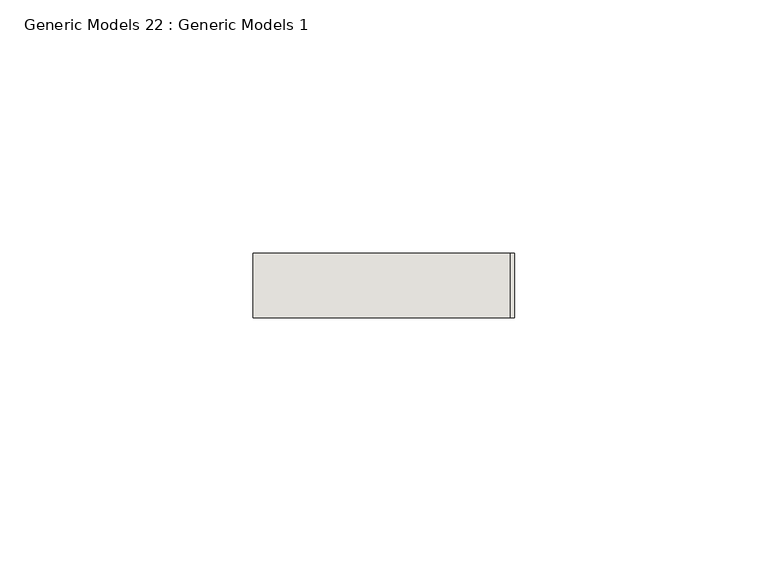
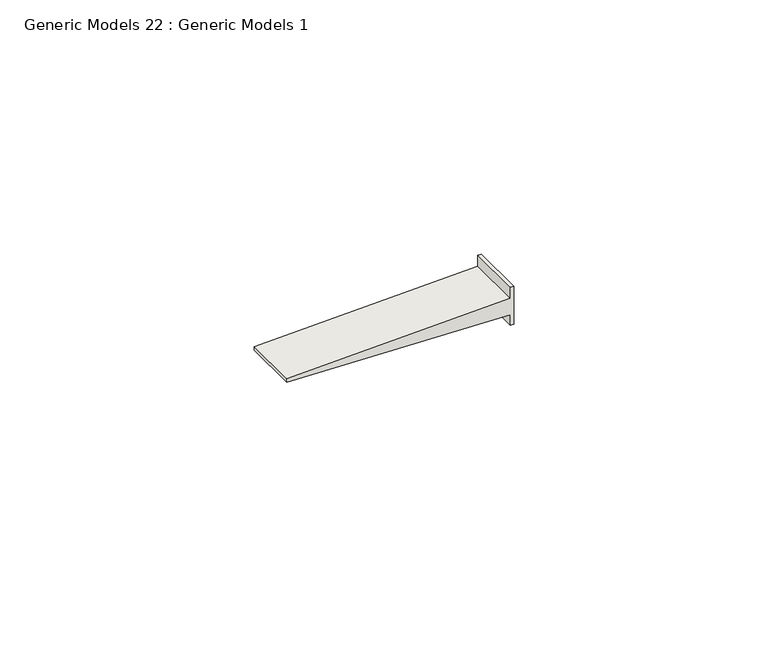
"""IFC4 building model written with IfcOpenShell, lengths in millimetres: wall geometry, Generic Models 22 : Generic Models 1."""

from ifc_helpers import new_model, si_unit, frame, origin, place, context, project, spatial, polyline, outline, extrude, source, transform, mapped, element, save


def generic_models_22_generic_models_1_082c1598(model_context):
    return source(origin(), model_context, "Body", "SweptSolid", [
        extrude(outline(polyline([(5490.9466, 49800.66875), (5490.9466, 49799.875), (5488.3967364, 49799.875), (5486.7993473, 49749.075), (5486.0006527, 49749.075), (5484.4032636, 49799.875), (5481.8534, 49799.875), (5481.8534, 49800.66875), (5490.9466, 49800.66875)])), frame((0.0, 565.15, 0.0), z_axis=(0.0, 1.0, 0.0), x_axis=(0.0, 0.0, 1.0)), (0.0, 0.0, 1.0), 12.7),
    ])


if __name__ == "__main__":
    model = new_model("IFC4")
    model_context = context("Model", 3, world=origin())
    ifc_project = project(units=[si_unit("LENGTHUNIT", "METRE", prefix="MILLI")], contexts=[model_context])
    site = spatial("IfcSite", under=ifc_project)
    building = spatial("IfcBuilding", under=site)
    placement = place(None, origin())
    generic_models_22_generic_models_1_shape = generic_models_22_generic_models_1_082c1598(model_context)
    element("IfcWall", 1, ObjectType="Generic Models 22 : Generic Models 1", at=placement, inside=building, context=model_context, shape_type="MappedRepresentation", body=[
        mapped(generic_models_22_generic_models_1_shape, transform((0.0, 0.0, 0.0), x_axis=(1.0, 0.0, 0.0), y_axis=(0.0, 1.0, 0.0), z_axis=(0.0, 0.0, 1.0))),
    ])
    save(model, "model.ifc")

# Revit data of these elements
# Element 1 (IfcWall, "Generic Models 22 : Generic Models 1")
#   Materials on its faces: "ATTACH GYPSUM BOARD TO STUDS AND NOT TO TOP TRACK"
# Materials
#   "ATTACH GYPSUM BOARD TO STUDS AND NOT TO TOP TRACK": class "Generic", colour RGB 48 48 48, transparency 0, Cost = 0
